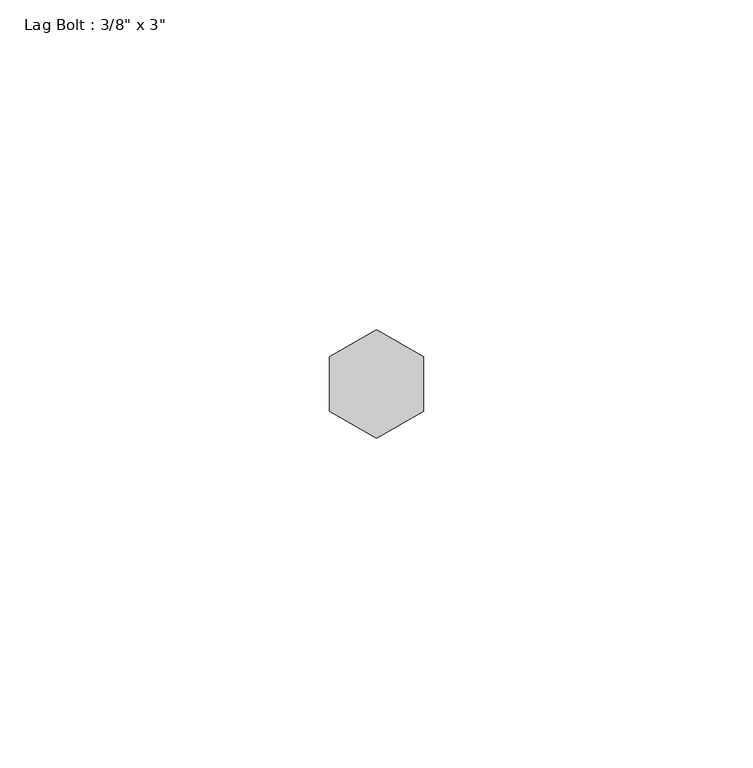
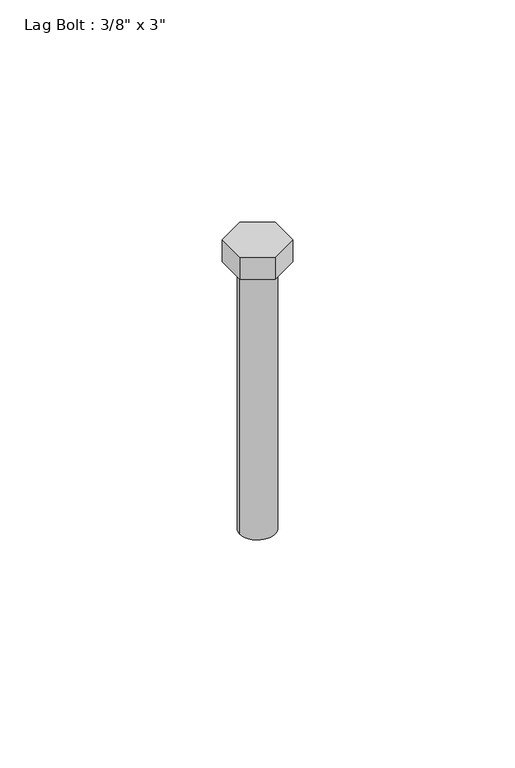
"""IFC4 building model written with IfcOpenShell, lengths in millimetres: proxy geometry."""

from ifc_helpers import new_model, si_unit, point, frame, origin, origin_with_axes, origin_2d, place, context, project, spatial, polyline, circle_curve, trimmed, segment, composite_curve, outline, extrude, source, transform, mapped, element, save


def proxy_911ead17(model_context):
    return source(origin(), model_context, "Body", "SweptSolid", [
        extrude(outline(polyline([(-7.14375, 4.124446), (0.0, 8.248892), (7.14375, 4.124446), (7.14375, -4.124446), (0.0, -8.248892), (-7.14375, -4.124446), (-7.14375, 4.124446)])), origin_with_axes(), (0.0, 0.0, 1.0), 6.35),
        extrude(outline(composite_curve([segment(trimmed(circle_curve(origin_2d(), 4.7625), [point((-4.7625, 0.0))], [point((4.7625, 0.0))], False, "CARTESIAN"), True, "CONTINUOUS"), segment(trimmed(circle_curve(origin_2d(), 4.7625), [point((4.7625, 0.0))], [point((-4.7625, 0.0))], False, "CARTESIAN"), True, "CONTINUOUS")], self_intersect=False)), frame((0.0, 0.0, -76.2), z_axis=(0.0, 0.0, 1.0), x_axis=(1.0, 0.0, 0.0)), (0.0, 0.0, 1.0), 76.2),
    ])


if __name__ == "__main__":
    model = new_model("IFC4")
    model_context = context("Model", 3, world=origin())
    ifc_project = project(units=[si_unit("LENGTHUNIT", "METRE", prefix="MILLI")], contexts=[model_context])
    site = spatial("IfcSite", under=ifc_project)
    building = spatial("IfcBuilding", under=site)
    placement = place(None, origin())
    proxy_shape = proxy_911ead17(model_context)
    element("IfcBuildingElementProxy", 1, Name="Lag Bolt : 3/8\" x 3\"", ObjectType="Lag Bolt : 3/8\" x 3\"", at=placement, inside=building, context=model_context, shape_type="MappedRepresentation", body=[
        mapped(proxy_shape, transform((0.0, 0.0, 0.0), x_axis=(1.0, 0.0, 0.0), y_axis=(0.0, 1.0, 0.0), z_axis=(0.0, 0.0, 1.0))),
    ])
    save(model, "model.ifc")

# Revit data of these elements
# Type "Lag Bolt : 3/8\" x 3\""
#   Thickness_of_Substrate [instance default] = 0' - 1"
#   Side = 0' - 0.3252"
#   Radius = 0' - 0 3/16"
#   Length = 0' - 3"
#   Head Size = 0' - 0 9/16"
#   Head Radius = 0' - 0 9/32"
#   Head Height = 0' - 0 1/4"
#   Diameter = 0' - 0 3/8"
#   Default Elevation = 4' - 0"
#   Nut_Visibility [instance default] = no
#   Bolt Material (Size) [instance default] = none
# Element 1 (IfcBuildingElementProxy, "Lag Bolt : 3/8\" x 3\"")
#   Bolt Material (Size) = _GALV. ANCHORS - SEE STRUCT. DWG
#   Materials on its faces: "_GALV. ANCHORS - SEE STRUCT. DWG"
# Materials
#   "_GALV. ANCHORS - SEE STRUCT. DWG": class "Generic", colour RGB 233 233 233, transparency 0, Cost = 0
